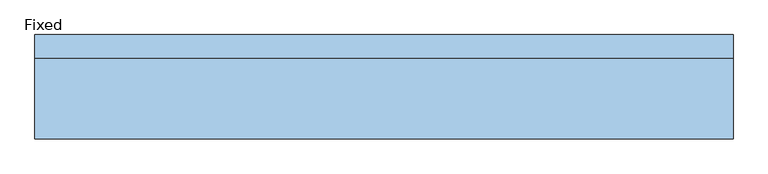
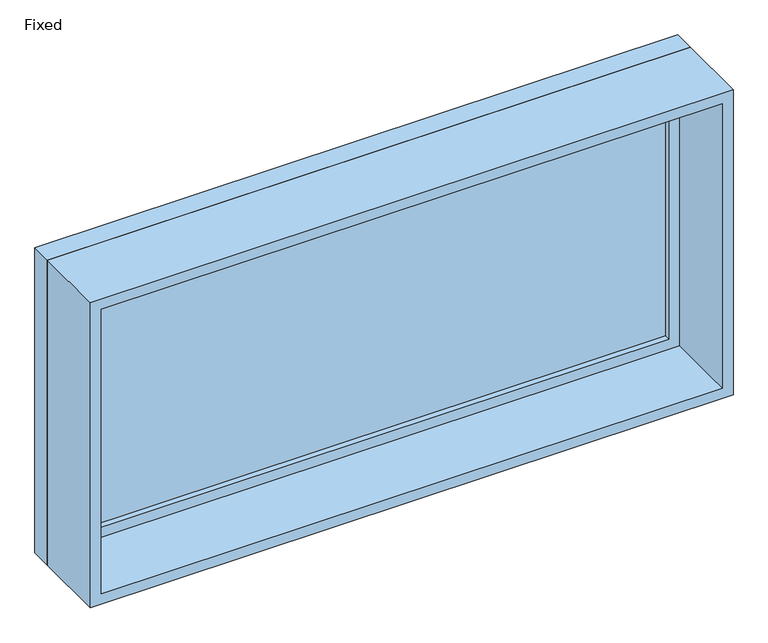
"""IFC4 building model written with IfcOpenShell, lengths in millimetres: window geometry, Fixed."""

from ifc_helpers import new_model, si_unit, frame, origin, place, context, project, spatial, polyline, outline, extrude, source, transform, mapped, element, save


def fixed_b37ba2c0(model_context):
    return source(origin(), model_context, "Body", "SweptSolid", [
        extrude(outline(polyline([(835.025, 92.075), (-911.225, 92.075), (-911.225, 104.775), (835.025, 104.775), (835.025, 92.075)])), frame((0.0, 0.0, 1257.3), z_axis=(0.0, 0.0, 1.0), x_axis=(1.0, 0.0, 0.0)), (0.0, 0.0, 1.0), 812.8),
        extrude(outline(polyline([(2114.55, -955.675), (1212.85, -955.675), (1212.85, 879.475), (2114.55, 879.475), (2114.55, -955.675)]), holes=[polyline([(2070.1, -911.225), (2070.1, 835.025), (1257.3, 835.025), (1257.3, -911.225), (2070.1, -911.225)])]), frame((0.0, 76.2, 0.0), z_axis=(0.0, 1.0, 0.0), x_axis=(0.0, 0.0, 1.0)), (0.0, 0.0, 1.0), 44.45),
        extrude(outline(polyline([(2133.6, -974.725), (1193.8, -974.725), (1193.8, 898.525), (2133.6, 898.525), (2133.6, -974.725)]), holes=[polyline([(2101.85, -942.975), (2101.85, 866.775), (1225.55, 866.775), (1225.55, -942.975), (2101.85, -942.975)])]), frame((0.0, -139.7, 0.0), z_axis=(0.0, 1.0, 0.0), x_axis=(0.0, 0.0, 1.0)), (0.0, 0.0, 1.0), 215.9),
        extrude(outline(polyline([(2133.6, 898.525), (2133.6, -974.725), (1193.8, -974.725), (1193.8, 898.525), (2133.6, 898.525)]), holes=[polyline([(2114.55, 879.475), (1212.85, 879.475), (1212.85, -955.675), (2114.55, -955.675), (2114.55, 879.475)])]), frame((0.0, 76.2, 0.0), z_axis=(0.0, 1.0, 0.0), x_axis=(0.0, 0.0, 1.0)), (0.0, 0.0, 1.0), 63.5),
    ])


if __name__ == "__main__":
    model = new_model("IFC4")
    model_context = context("Model", 3, world=origin())
    ifc_project = project(units=[si_unit("LENGTHUNIT", "METRE", prefix="MILLI")], contexts=[model_context])
    site = spatial("IfcSite", under=ifc_project)
    building = spatial("IfcBuilding", under=site)
    placement = place(None, origin())
    fixed_shape = fixed_b37ba2c0(model_context)
    element("IfcWindow", 1, ObjectType="Fixed : 6' 1 34\"\" x 3' 1\"", at=placement, inside=building, context=model_context, shape_type="MappedRepresentation", body=[
        mapped(fixed_shape, transform((0.0, 0.0, 0.0), x_axis=(1.0, 0.0, 0.0), y_axis=(0.0, 1.0, 0.0), z_axis=(0.0, 0.0, 1.0))),
    ])
    save(model, "model.ifc")

# Revit data of these elements
# Type "Fixed : 6' 1 34\"\" x 3' 1\""
#   Type Mark = "10"
#   Assembly Code = "B2020100"
#   Height = 3' - 1"
#   Default Sill Height = 3' - 11"
#   Width = 6' - 1 3/4"
#   Window Inset = 0' - 0 3/4"
#   Glass Pane Material = Glass
#   Sash Material = accent 2
#   Wall Closure = (empty or 0)
# Element 1 (IfcWindow, "Fixed : 6' 1 34\"\" x 3' 1\"")
#   Materials on its faces: "accent 2", "Glass"
# Materials
#   "Glass": class "Glass", colour RGB 236 240 239, transparency 0.85, Description = "Soda Lime Glass", Cost = 0
#   "accent 2": class "Wood", colour RGB 80 80 80, transparency 0, Description = "Wood framing, thermal airspace", Cost = 0
